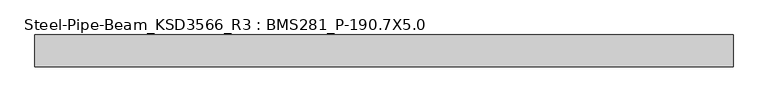
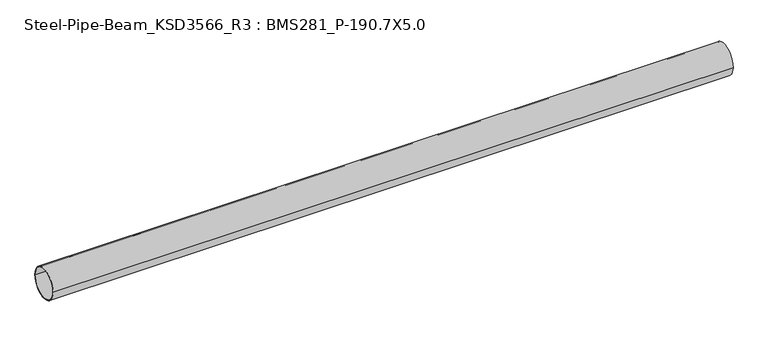
"""IFC4 building model written with IfcOpenShell, lengths in millimetres: member geometry, Steel-Pipe-Beam_KSD3566_R3 : BMS281_P-190.7X5.0."""

from ifc_helpers import new_model, si_unit, point, frame, origin, origin_2d, place, context, project, spatial, circle_curve, trimmed, segment, composite_curve, outline, extrude, source, transform, mapped, element, save


def steel_pipe_beam_ksd3566_r3_bms281_p_190_7x5_0_348ae839(model_context):
    return source(origin(), model_context, "Body", "SweptSolid", [
        extrude(outline(composite_curve([segment(trimmed(circle_curve(origin_2d(), 95.35), [point((-95.35, 0.0))], [point((95.35, 0.0))], False, "CARTESIAN"), True, "CONTINUOUS"), segment(trimmed(circle_curve(origin_2d(), 95.35), [point((95.35, 0.0))], [point((-95.35, 0.0))], False, "CARTESIAN"), True, "CONTINUOUS")], self_intersect=False), holes=[composite_curve([segment(trimmed(circle_curve(origin_2d(), 90.35), [point((90.35, 0.0))], [point((-90.35, 0.0))], True, "CARTESIAN"), True, "CONTINUOUS"), segment(trimmed(circle_curve(origin_2d(), 90.35), [point((-90.35, 0.0))], [point((90.35, 0.0))], True, "CARTESIAN"), True, "CONTINUOUS")], self_intersect=False)]), frame((-2046.1374086, 0.0, 0.0), z_axis=(1.0, 0.0, 0.0), x_axis=(0.0, 1.0, 0.0)), (0.0, 0.0, 1.0), 4152.4090653),
    ])


if __name__ == "__main__":
    model = new_model("IFC4")
    model_context = context("Model", 3, world=origin())
    ifc_project = project(units=[si_unit("LENGTHUNIT", "METRE", prefix="MILLI")], contexts=[model_context])
    site = spatial("IfcSite", under=ifc_project)
    building = spatial("IfcBuilding", under=site)
    placement = place(None, origin())
    steel_pipe_beam_ksd3566_r3_bms281_p_190_7x5_0_shape = steel_pipe_beam_ksd3566_r3_bms281_p_190_7x5_0_348ae839(model_context)
    element("IfcMember", 1, ObjectType="Steel-Pipe-Beam_KSD3566_R3 : BMS281_P-190.7X5.0", at=placement, inside=building, context=model_context, shape_type="MappedRepresentation", body=[
        mapped(steel_pipe_beam_ksd3566_r3_bms281_p_190_7x5_0_shape, transform((0.0, 0.0, 0.0), x_axis=(1.0, 0.0, 0.0), y_axis=(0.0, 1.0, 0.0), z_axis=(0.0, 0.0, 1.0))),
    ])
    save(model, "model.ifc")

# Revit data of these elements
# Type "Steel-Pipe-Beam_KSD3566_R3 : BMS281_P-190.7X5.0"
#   Keynote = "P-190.7X5.0"
#   SteelWeight = "Light"
#   t = 0.0050 m
#   Surface Area = 0.599102 m²/m
#   Section Area = 29.1697 cm²
#   Mass per Unit Length = 22.8982 kg/m
#   Length [instance default] = 1.5000 m
#   D = 0.1907 m
#   hec_material4 [instance default] = none
#   hec_material3 [instance default] = none
#   hec_material2 [instance default] = none
#   hec_material1 [instance default] = none
#   Structural Material [instance default] = Steel, 45-345
#   Assembly Code = ""
# Element 1 (IfcMember, "Steel-Pipe-Beam_KSD3566_R3 : BMS281_P-190.7X5.0")
#   Structural Material = none
# Materials
#   "Steel, 45-345": class "Metal", colour RGB 189 187 185, transparency 0, Description = "Steel 345 MPa", Cost = 0
